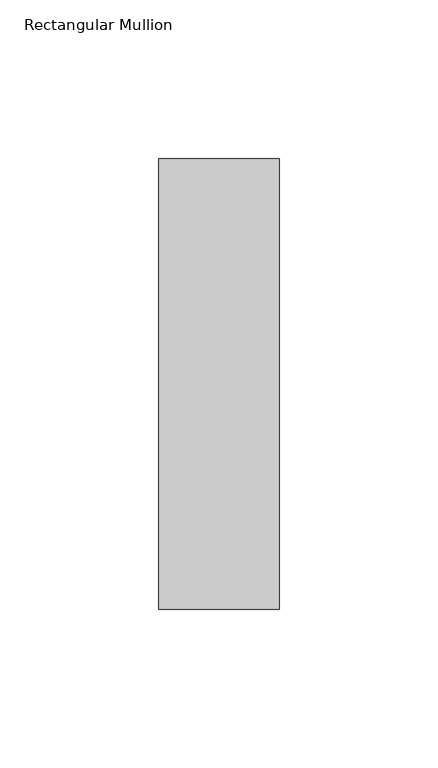
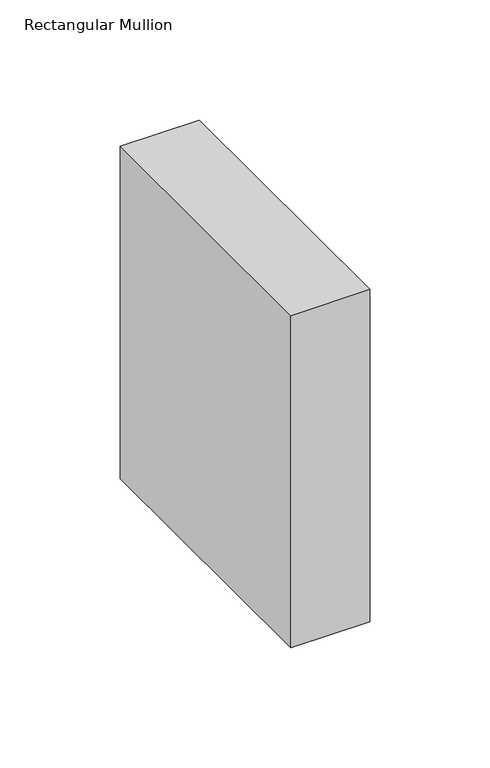
"""IFC4 building model written with IfcOpenShell, lengths in millimetres: member geometry, Rectangular Mullion : NLRS_21_CWM_hsb-regel 38x142_gen_rsf."""

from ifc_helpers import new_model, si_unit, frame, origin, place, context, project, spatial, polyline, outline, extrude, source, transform, mapped, element, save


def rectangular_mullion_fbae096f(model_context):
    return source(origin(), model_context, "Body", "SweptSolid", [
        extrude(outline(polyline([(-38.0, -71.0), (-38.0, 71.0), (0.0, 71.0), (0.0, -71.0), (-38.0, -71.0)])), frame((0.0, 0.0, -168.9999997), z_axis=(0.0, 0.0, 1.0), x_axis=(1.0, 0.0, 0.0)), (0.0, 0.0, 1.0), 168.9999997),
    ])


if __name__ == "__main__":
    model = new_model("IFC4")
    model_context = context("Model", 3, world=origin())
    ifc_project = project(units=[si_unit("LENGTHUNIT", "METRE", prefix="MILLI")], contexts=[model_context])
    site = spatial("IfcSite", under=ifc_project)
    building = spatial("IfcBuilding", under=site)
    placement = place(None, origin())
    rectangular_mullion_shape = rectangular_mullion_fbae096f(model_context)
    element("IfcMember", 1, ObjectType="Rectangular Mullion : NLRS_21_CWM_hsb-regel 38x142_gen_rsf", at=placement, inside=building, context=model_context, shape_type="MappedRepresentation", body=[
        mapped(rectangular_mullion_shape, transform((0.0, 0.0, 0.0), x_axis=(1.0, 0.0, 0.0), y_axis=(0.0, 1.0, 0.0), z_axis=(0.0, 0.0, 1.0))),
    ])
    save(model, "model.ifc")

# Revit data of these elements
# Type "Rectangular Mullion : NLRS_21_CWM_hsb-regel 38x142_gen_rsf"
#   Export Type to IFC As = "IfcWall"
#   Type IfcGUID = "07M7mRoiH1CR8m_RSKIwpF"
#   Assembly Code = "21.10"
#   built-in parameter 1007322 = 0.465879 (stored number, unit not read)
#   built-in parameter 1007321 = 0.062336 (stored number, unit not read)
#   built-in parameter 1007320 = 0.062336 (stored number, unit not read)
# Element 1 (IfcMember, "Rectangular Mullion : NLRS_21_CWM_hsb-regel 38x142_gen_rsf")
#   Materials on its faces: "NLRS_i2_hout naaldhout vuren_gen_rsf"
# Materials
#   "NLRS_i2_hout naaldhout vuren_gen_rsf": class "I - Hout", colour RGB 234 199 147, transparency 0, Keynote = "i2", Manufacturer = "Revit Standards Foundation", URL = "www.revitstandards.org", Description = "hout vuren", Cost = 0
